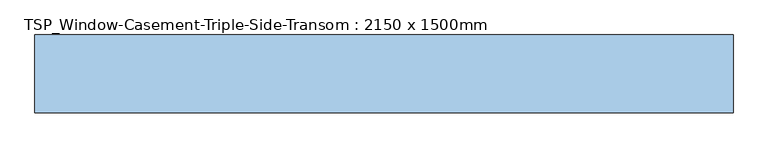
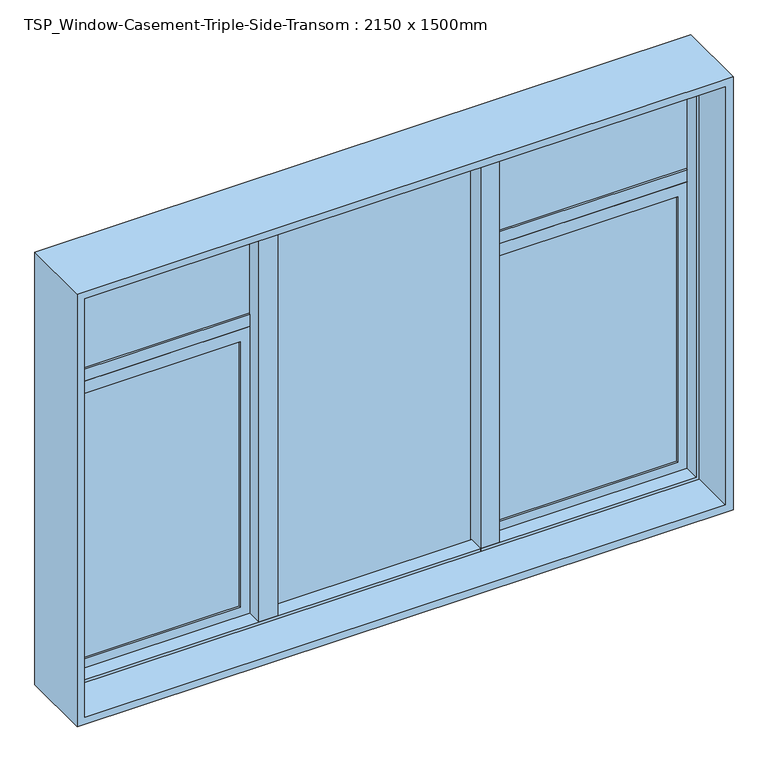
"""IFC4 building model written with IfcOpenShell, lengths in millimetres: window geometry, TSP_Window-Casement-Triple-Side-Transom : 2150 x 1500mm."""

from ifc_helpers import new_model, si_unit, frame, origin, place, context, project, spatial, polyline, outline, extrude, faceted_brep, source, transform, mapped, element, save


def tsp_window_casement_triple_side_transom_2150_x_1500mm_17097b4f(model_context):
    return source(origin(), model_context, "Body", "SolidModel", [
        faceted_brep([(-1049.6, 78.725, 2374.6), (-1049.6, 120.025, 2374.6), (1049.6, 120.025, 2374.6), (1049.6, 78.725, 2374.6), (-1039.5, 27.925, 2364.5), (-1039.5, 78.725, 2364.5), (1039.5, 78.725, 2364.5), (1039.5, 27.925, 2364.5), (-1049.6, -120.0, 2374.6), (-1049.6, 27.925, 2374.6), (1049.6, 27.925, 2374.6), (1049.6, -120.0, 2374.6), (-1075.0, 120.025, 2400.0), (-1075.0, -120.0, 2400.0), (1075.0, -120.0, 2400.0), (1075.0, 120.025, 2400.0), (1049.6, 120.025, 925.4), (1049.6, 78.725, 925.4), (1039.5, 78.725, 935.5), (1039.5, 27.925, 935.5), (1049.6, 27.925, 925.4), (1049.6, -120.0, 925.4), (1075.0, -120.0, 900.0), (1075.0, 120.025, 900.0), (-1049.6, 120.025, 925.4), (-1049.6, 78.725, 925.4), (-1039.5, 78.725, 935.5), (-1039.5, 27.925, 935.5), (-1049.6, 27.925, 925.4), (-1049.6, -120.0, 925.4), (-1075.0, -120.0, 900.0), (-1075.0, 120.025, 900.0)], [[[0, 1, 2, 3]], [[4, 5, 6, 7]], [[8, 9, 10, 11]], [[12, 13, 14, 15]], [[3, 2, 16, 17]], [[7, 6, 18, 19]], [[11, 10, 20, 21]], [[15, 14, 22, 23]], [[17, 16, 24, 25]], [[19, 18, 26, 27]], [[21, 20, 28, 29]], [[23, 22, 30, 31]], [[25, 24, 1, 0]], [[3, 17, 25, 0], [5, 26, 18, 6]], [[27, 26, 5, 4]], [[9, 28, 20, 10], [7, 19, 27, 4]], [[29, 28, 9, 8]], [[13, 30, 22, 14], [11, 21, 29, 8]], [[31, 30, 13, 12]], [[15, 23, 31, 12], [1, 24, 16, 2]]]),
        extrude(outline(polyline([(-332.9333333, 116.825), (-332.9333333, 27.925), (-393.8333333, 27.925), (-393.8333333, 78.725), (-383.7333333, 78.725), (-383.7333333, 116.825), (-332.9333333, 116.825)])), frame((0.0, 0.0, 925.4), z_axis=(0.0, 0.0, 1.0), x_axis=(1.0, 0.0, 0.0)), (0.0, 0.0, 1.0), 1449.2),
        extrude(outline(polyline([(383.7333333, 116.825), (383.7333333, 78.725), (393.8333333, 78.725), (393.8333333, 27.925), (332.9333333, 27.925), (332.9333333, 116.825), (383.7333333, 116.825)])), frame((0.0, 0.0, 925.4), z_axis=(0.0, 0.0, 1.0), x_axis=(1.0, 0.0, 0.0)), (0.0, 0.0, 1.0), 1449.2),
        extrude(outline(polyline([(1929.05, 383.7333333), (925.4, 383.7333333), (925.4, 1049.6), (1929.05, 1049.6), (1929.05, 383.7333333)]), holes=[polyline([(1887.15, 1007.7), (967.3, 1007.7), (967.3, 425.6333333), (1887.15, 425.6333333), (1887.15, 1007.7)])]), frame((0.0, 78.725, 0.0), z_axis=(0.0, 1.0, 0.0), x_axis=(0.0, 0.0, 1.0)), (0.0, 0.0, 1.0), 31.75),
        extrude(outline(polyline([(1929.05, -1049.6), (925.4, -1049.6), (925.4, -383.7333333), (1929.05, -383.7333333), (1929.05, -1049.6)]), holes=[polyline([(1887.15, -425.6333333), (967.3, -425.6333333), (967.3, -1007.7), (1887.15, -1007.7), (1887.15, -425.6333333)])]), frame((0.0, 78.725, 0.0), z_axis=(0.0, 1.0, 0.0), x_axis=(0.0, 0.0, 1.0)), (0.0, 0.0, 1.0), 31.75),
        extrude(outline(polyline([(-425.6333333, 104.125), (-425.6333333, 97.775), (-1007.7, 97.775), (-1007.7, 104.125), (-425.6333333, 104.125)])), frame((0.0, 0.0, 967.3), z_axis=(0.0, 0.0, 1.0), x_axis=(1.0, 0.0, 0.0)), (0.0, 0.0, 1.0), 919.85),
        extrude(outline(polyline([(-425.6333333, 91.425), (-425.6333333, 85.075), (-1007.7, 85.075), (-1007.7, 91.425), (-425.6333333, 91.425)])), frame((0.0, 0.0, 967.3), z_axis=(0.0, 0.0, 1.0), x_axis=(1.0, 0.0, 0.0)), (0.0, 0.0, 1.0), 919.85),
        extrude(outline(polyline([(1007.7, 104.125), (1007.7, 97.775), (425.6333333, 97.775), (425.6333333, 104.125), (1007.7, 104.125)])), frame((0.0, 0.0, 967.3), z_axis=(0.0, 0.0, 1.0), x_axis=(1.0, 0.0, 0.0)), (0.0, 0.0, 1.0), 919.85),
        extrude(outline(polyline([(1007.7, 91.425), (1007.7, 85.075), (425.6333333, 85.075), (425.6333333, 91.425), (1007.7, 91.425)])), frame((0.0, 0.0, 967.3), z_axis=(0.0, 0.0, 1.0), x_axis=(1.0, 0.0, 0.0)), (0.0, 0.0, 1.0), 919.85),
        extrude(outline(polyline([(1049.6, 110.475), (1049.6, 78.725), (383.7333333, 78.725), (383.7333333, 110.475), (1049.6, 110.475)])), frame((0.0, 0.0, 1929.05), z_axis=(0.0, 0.0, 1.0), x_axis=(1.0, 0.0, 0.0)), (0.0, 0.0, 1.0), 41.9),
        extrude(outline(polyline([(332.9333333, 104.125), (332.9333333, 97.775), (-332.9333333, 97.775), (-332.9333333, 104.125), (332.9333333, 104.125)])), frame((0.0, 0.0, 925.4), z_axis=(0.0, 0.0, 1.0), x_axis=(1.0, 0.0, 0.0)), (0.0, 0.0, 1.0), 1449.2),
        extrude(outline(polyline([(332.9333333, 91.425), (332.9333333, 85.075), (-332.9333333, 85.075), (-332.9333333, 91.425), (332.9333333, 91.425)])), frame((0.0, 0.0, 925.4), z_axis=(0.0, 0.0, 1.0), x_axis=(1.0, 0.0, 0.0)), (0.0, 0.0, 1.0), 1449.2),
        extrude(outline(polyline([(-383.7333333, 110.475), (-383.7333333, 78.725), (-1049.6, 78.725), (-1049.6, 110.475), (-383.7333333, 110.475)])), frame((0.0, 0.0, 1929.05), z_axis=(0.0, 0.0, 1.0), x_axis=(1.0, 0.0, 0.0)), (0.0, 0.0, 1.0), 41.9),
        extrude(outline(polyline([(-383.7333333, 104.125), (-383.7333333, 97.775), (-1049.6, 97.775), (-1049.6, 104.125), (-383.7333333, 104.125)])), frame((0.0, 0.0, 1970.95), z_axis=(0.0, 0.0, 1.0), x_axis=(1.0, 0.0, 0.0)), (0.0, 0.0, 1.0), 403.65),
        extrude(outline(polyline([(-383.7333333, 91.425), (-383.7333333, 85.075), (-1049.6, 85.075), (-1049.6, 91.425), (-383.7333333, 91.425)])), frame((0.0, 0.0, 1970.95), z_axis=(0.0, 0.0, 1.0), x_axis=(1.0, 0.0, 0.0)), (0.0, 0.0, 1.0), 403.65),
        extrude(outline(polyline([(1049.6, 104.125), (1049.6, 97.775), (383.7333333, 97.775), (383.7333333, 104.125), (1049.6, 104.125)])), frame((0.0, 0.0, 1970.95), z_axis=(0.0, 0.0, 1.0), x_axis=(1.0, 0.0, 0.0)), (0.0, 0.0, 1.0), 403.65),
        extrude(outline(polyline([(1049.6, 91.425), (1049.6, 85.075), (383.7333333, 85.075), (383.7333333, 91.425), (1049.6, 91.425)])), frame((0.0, 0.0, 1970.95), z_axis=(0.0, 0.0, 1.0), x_axis=(1.0, 0.0, 0.0)), (0.0, 0.0, 1.0), 403.65),
    ])


if __name__ == "__main__":
    model = new_model("IFC4")
    model_context = context("Model", 3, world=origin())
    ifc_project = project(units=[si_unit("LENGTHUNIT", "METRE", prefix="MILLI")], contexts=[model_context])
    site = spatial("IfcSite", under=ifc_project)
    building = spatial("IfcBuilding", under=site)
    placement = place(None, origin())
    tsp_window_casement_triple_side_transom_2150_x_1500mm_shape = tsp_window_casement_triple_side_transom_2150_x_1500mm_17097b4f(model_context)
    element("IfcWindow", 1, ObjectType="TSP_Window-Casement-Triple-Side-Transom : 2150 x 1500mm", at=placement, inside=building, context=model_context, shape_type="MappedRepresentation", body=[
        mapped(tsp_window_casement_triple_side_transom_2150_x_1500mm_shape, transform((0.0, 0.0, 0.0), x_axis=(1.0, 0.0, 0.0), y_axis=(0.0, 1.0, 0.0), z_axis=(0.0, 0.0, 1.0))),
    ])
    save(model, "model.ifc")

# Revit data of these elements
# Type "TSP_Window-Casement-Triple-Side-Transom : 2150 x 1500mm"
#   Type Mark = "HS 2412 F36"
#   Fire Rating = "0.5h"
#   Assembly Code = "B2020100"
#   Analytic Construction = "Double glazing - domestic"
#   Window Width = 716.667 mm
#   Window Inset [instance default] = 15.875 mm
#   Wall Thickness [instance default] = 150 mm
#   Visual Light Transmittance = 0.81
#   Transom Height Ratio = 0.3
#   Thermal Resistance (R) = 0.319569 (m²·K)/W
#   Solar Heat Gain Coefficient = 0.76
#   Rough Width = 2165 mm
#   Rough Height = 1515 mm
#   Open Window Height = 1050 mm
#   Heat Transfer Coefficient (U) = 3.12929 W/(m²·K)
#   Height = 1500 mm
#   Transom Height = 450 mm
#   Frame Gap 3 [instance default] = 41.9 mm
#   Frame Gap 2 [instance default] = 15.9 mm
#   Frame Gap 1 = 35.5 mm
#   Default Sill Height = 900 mm
#   Width = 2150 mm
#   Frame Material = Metal - Aluminum
#   Glass Panel Material = Glass
#   Wall Closure = (empty or 0)
# Element 1 (IfcWindow, "TSP_Window-Casement-Triple-Side-Transom : 2150 x 1500mm")
#   Wall Thickness = 240 mm
#   Materials on its faces: "Metal - Aluminum", "Glass"
# Materials
#   "Metal - Aluminum": class "Metal", colour RGB 247 247 247, transparency 0
#   "Glass": class "Glass", colour RGB 0 128 192, transparency 0.9, Description = "Soda Lime Glass", Cost = 0
